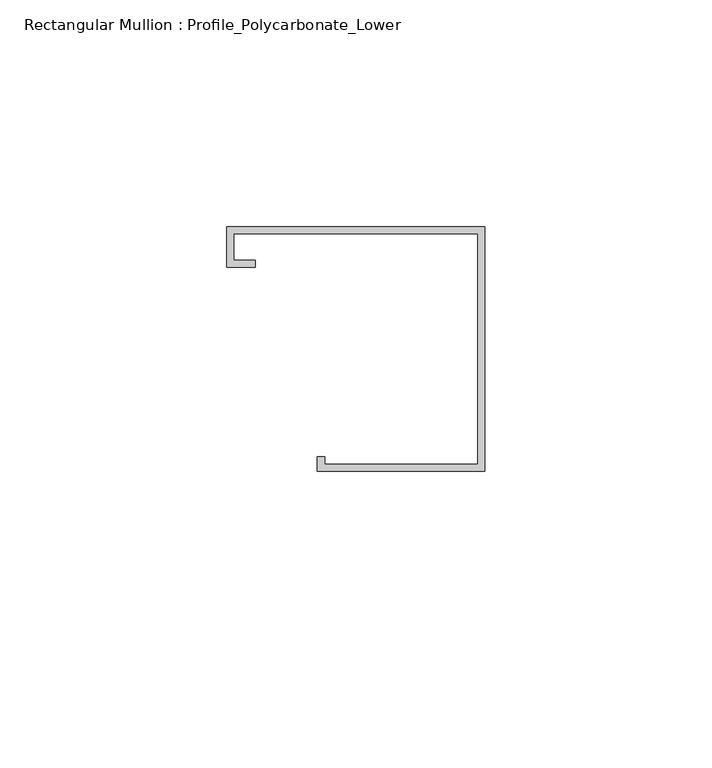
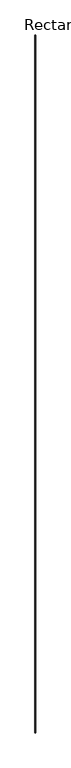
"""IFC4 building model written with IfcOpenShell, lengths in millimetres: member geometry, Rectangular Mullion : Profile_Polycarbonate_Lower."""

from ifc_helpers import new_model, si_unit, frame, origin, place, context, project, spatial, polyline, outline, extrude, source, transform, mapped, element, save


def rectangular_mullion_profile_polycarbonate_lower_753cb222(model_context):
    return source(origin(), model_context, "Body", "SweptSolid", [
        extrude(outline(polyline([(0.0, 28.984575), (0.0, -25.015825), (-36.9824, -25.015825), (-36.9824, -21.840825), (-35.3949, -21.840825), (-35.3949, -23.428325), (-1.5875, -23.428325), (-1.5875, 27.397075), (-55.4101, 27.397075), (-55.4101, 21.580475), (-50.6476, 21.580475), (-50.6476, 19.992975), (-56.9976, 19.992975), (-56.9976, 28.984575), (0.0, 28.984575)])), frame((0.0, 0.0, -88474.677), z_axis=(0.0, 0.0, 1.0), x_axis=(1.0, 0.0, 0.0)), (0.0, 0.0, 1.0), 88474.677),
    ])


if __name__ == "__main__":
    model = new_model("IFC4")
    model_context = context("Model", 3, world=origin())
    ifc_project = project(units=[si_unit("LENGTHUNIT", "METRE", prefix="MILLI")], contexts=[model_context])
    site = spatial("IfcSite", under=ifc_project)
    building = spatial("IfcBuilding", under=site)
    placement = place(None, origin())
    rectangular_mullion_profile_polycarbonate_lower_shape = rectangular_mullion_profile_polycarbonate_lower_753cb222(model_context)
    element("IfcMember", 1, ObjectType="Rectangular Mullion : Profile_Polycarbonate_Lower", at=placement, inside=building, context=model_context, shape_type="MappedRepresentation", body=[
        mapped(rectangular_mullion_profile_polycarbonate_lower_shape, transform((0.0, 0.0, 0.0), x_axis=(1.0, 0.0, 0.0), y_axis=(0.0, 1.0, 0.0), z_axis=(0.0, 0.0, 1.0))),
    ])
    save(model, "model.ifc")

# Revit data of these elements
# Type "Rectangular Mullion : Profile_Polycarbonate_Lower"
#   built-in parameter 1007322 = 0.177167 (stored number, unit not read)
#   built-in parameter 1007321 = 0 (stored number, unit not read)
#   built-in parameter 1007320 = 0.00520833 (stored number, unit not read)
